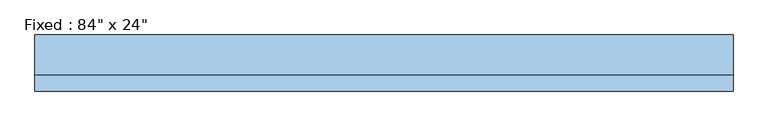
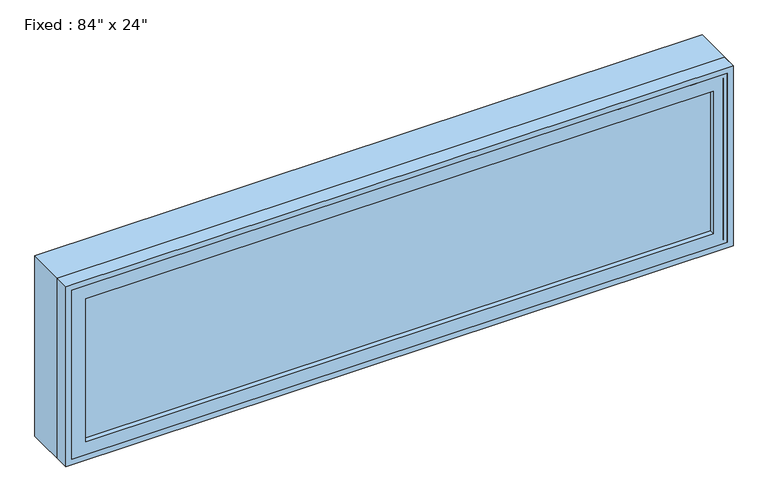
"""IFC4 building model written with IfcOpenShell, lengths in millimetres: window geometry."""

from ifc_helpers import new_model, si_unit, frame, origin, place, context, project, spatial, polyline, outline, extrude, source, transform, mapped, element, save


def window_8fe3d2ed(model_context):
    return source(origin(), model_context, "Body", "SweptSolid", [
        extrude(outline(polyline([(965.2, -93.6625), (-1041.4, -93.6625), (-1041.4, -80.9625), (965.2, -80.9625), (965.2, -93.6625)])), frame((0.0, 0.0, 1282.7), z_axis=(0.0, 0.0, 1.0), x_axis=(1.0, 0.0, 0.0)), (0.0, 0.0, 1.0), 482.6),
        extrude(outline(polyline([(1809.75, -1085.85), (1238.25, -1085.85), (1238.25, 1009.65), (1809.75, 1009.65), (1809.75, -1085.85)]), holes=[polyline([(1765.3, -1041.4), (1765.3, 965.2), (1282.7, 965.2), (1282.7, -1041.4), (1765.3, -1041.4)])]), frame((0.0, -109.5375, 0.0), z_axis=(0.0, 1.0, 0.0), x_axis=(0.0, 0.0, 1.0)), (0.0, 0.0, 1.0), 44.45),
        extrude(outline(polyline([(1828.8, -1104.9), (1219.2, -1104.9), (1219.2, 1028.7), (1828.8, 1028.7), (1828.8, -1104.9)]), holes=[polyline([(1797.05, -1073.15), (1797.05, 996.95), (1250.95, 996.95), (1250.95, -1073.15), (1797.05, -1073.15)])]), frame((0.0, -109.5375, 0.0), z_axis=(0.0, 1.0, 0.0), x_axis=(0.0, 0.0, 1.0)), (0.0, 0.0, 1.0), 47.625),
        extrude(outline(polyline([(1828.8, 1028.7), (1828.8, -1104.9), (1219.2, -1104.9), (1219.2, 1028.7), (1828.8, 1028.7)]), holes=[polyline([(1809.75, 1009.65), (1238.25, 1009.65), (1238.25, -1085.85), (1809.75, -1085.85), (1809.75, 1009.65)])]), frame((0.0, -109.5375, 0.0), z_axis=(0.0, 1.0, 0.0), x_axis=(0.0, 0.0, 1.0)), (0.0, 0.0, 1.0), 171.45),
    ])


if __name__ == "__main__":
    model = new_model("IFC4")
    model_context = context("Model", 3, world=origin())
    ifc_project = project(units=[si_unit("LENGTHUNIT", "METRE", prefix="MILLI")], contexts=[model_context])
    site = spatial("IfcSite", under=ifc_project)
    building = spatial("IfcBuilding", under=site)
    placement = place(None, origin())
    window_shape = window_8fe3d2ed(model_context)
    element("IfcWindow", 1, ObjectType="Fixed : 84\" x 24\"", at=placement, inside=building, context=model_context, shape_type="MappedRepresentation", body=[
        mapped(window_shape, transform((0.0, 0.0, 0.0), x_axis=(1.0, 0.0, 0.0), y_axis=(0.0, 1.0, 0.0), z_axis=(0.0, 0.0, 1.0))),
    ])
    save(model, "model.ifc")

# Revit data of these elements
# Type "Fixed : 84\" x 24\""
#   Type Mark = "20"
#   Construction Type Id = "GSP4R"
#   Assembly Code = "B2020100"
#   Analytic Construction = "1/8 in Pilkington single glazing"
#   Visual Light Transmittance = 0.9
#   Solar Heat Gain Coefficient = 0.78
#   Heat Transfer Coefficient (U) = 3.6886 W/(m²·K)
#   Height = 2' - 0"
#   Default Sill Height = 4' - 0"
#   Width = 7' - 0"
#   Window Inset = 0' - 5"
#   Glass Pane Material = Glass
#   Sash Material = Sash
#   Wall Closure = (empty or 0)
# Element 1 (IfcWindow, "Fixed : 84\" x 24\"")
#   Materials on its faces: "Sash", "Glass"
# Materials
#   "Glass": class "Glass", colour RGB 0 128 192, transparency 0.75, Description = "Soda Lime Glass", Cost = 0
#   "Sash": class "Wood", colour RGB 224 178 126, transparency 0
